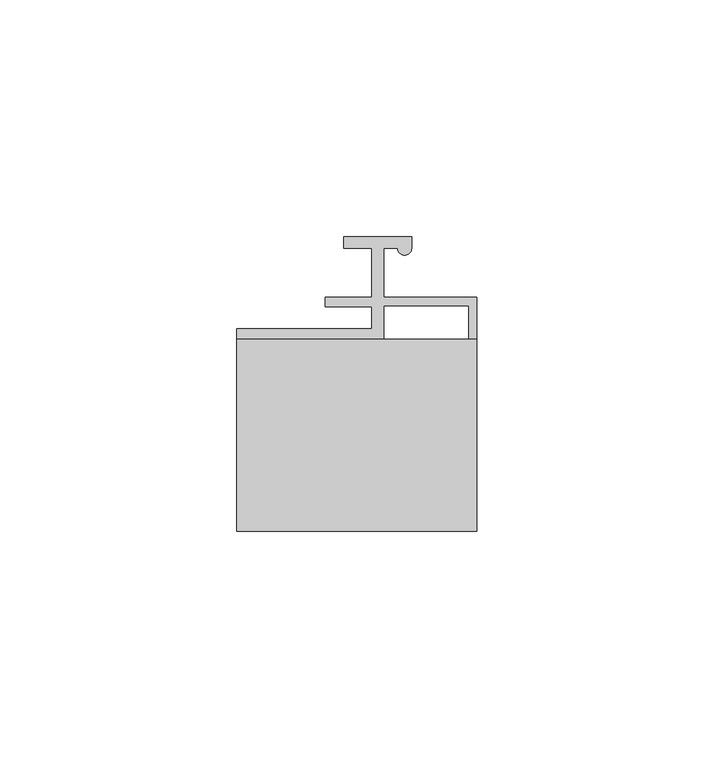
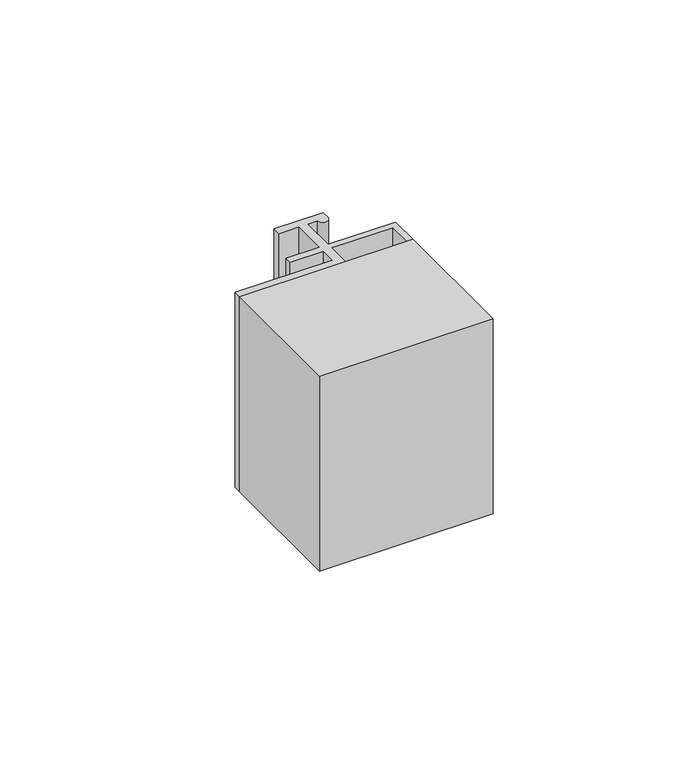
"""IFC4 building model written with IfcOpenShell, lengths in millimetres: proxy geometry, Generic Models 9:Generic Models 5:348123:Generic Models 5:348123 : Generic Models 9:Generic Models 5:348123:1 : Generic Models 9:Generic Models 5:348123:Generic Models 5:348123 : Generic Models 9:Generic Models 5:348123:301771."""

from ifc_helpers import new_model, si_unit, point, frame, frame_2d, origin, place, context, project, spatial, polyline, circle_curve, trimmed, segment, composite_curve, outline, extrude, source, transform, mapped, element, save


def generic_models_7091c7e3(model_context):
    return source(origin(), model_context, "Body", "SweptSolid", [
        extrude(outline(polyline([(30803.1241035, 40787.9731612), (30803.1241035, 40828.5678214), (30853.9241035, 40828.5678214), (30853.9241035, 40787.9731612), (30803.1241035, 40787.9731612)])), frame((0.0, 0.0, 267387.3875), z_axis=(0.0, 0.0, 1.0), x_axis=(1.0, 0.0, 0.0)), (0.0, 0.0, 1.0), 60.325),
        extrude(outline(composite_curve([segment(polyline([(30834.1959481, 40837.4454913), (30853.9241035, 40837.4454913), (30853.9241035, 40828.5678214), (30852.1485695, 40828.5678214), (30852.1485695, 40835.6699573), (30834.1959481, 40835.6699573), (30834.1959481, 40828.5678214), (30803.1241035, 40828.5678214), (30803.1241035, 40830.8365593), (30831.7299287, 40830.8365593), (30831.7299287, 40835.4726758), (30821.8658511, 40835.4726758), (30821.8658511, 40837.4454913), (30831.7299287, 40837.4454913), (30831.7299287, 40847.8027728), (30825.8114821, 40847.8027728), (30825.8114821, 40850.2687923), (30840.1143948, 40850.2687923), (30840.1143948, 40847.8027728)]), True, "CONTINUOUS"), segment(trimmed(circle_curve(frame_2d((30838.6347831, 40847.8027728)), 1.4796117), [point((30840.1143948, 40847.8027728))], [point((30837.1551714, 40847.8027728))], False, "CARTESIAN"), True, "CONTINUOUS"), segment(polyline([(30837.1551714, 40847.8027728), (30834.1959481, 40847.8027728), (30834.1959481, 40837.4454913)]), True, "CONTINUOUS")], self_intersect=False)), frame((0.0, 0.0, 267387.3875), z_axis=(0.0, 0.0, 1.0), x_axis=(1.0, 0.0, 0.0)), (0.0, 0.0, 1.0), 60.325),
    ])


if __name__ == "__main__":
    model = new_model("IFC4")
    model_context = context("Model", 3, world=origin())
    ifc_project = project(units=[si_unit("LENGTHUNIT", "METRE", prefix="MILLI")], contexts=[model_context])
    site = spatial("IfcSite", under=ifc_project)
    building = spatial("IfcBuilding", under=site)
    placement = place(None, origin())
    generic_models_shape = generic_models_7091c7e3(model_context)
    element("IfcBuildingElementProxy", 1, Name="Generic Models 9:Generic Models 5:348123:Generic Models 5:348123 : Generic Models 9:Generic Models 5:348123:1 : Generic Models 9:Generic Models 5:348123:Generic Models 5:348123 : Generic Models 9:Generic Models 5:348123:301771", ObjectType="Generic Models 9:Generic Models 5:348123:Generic Models 5:348123 : Generic Models 9:Generic Models 5:348123:1 : Generic Models 9:Generic Models 5:348123:Generic Models 5:348123 : Generic Models 9:Generic Models 5:348123:301771", at=placement, inside=building, context=model_context, shape_type="MappedRepresentation", body=[
        mapped(generic_models_shape, transform((0.0, 0.0, 0.0), x_axis=(1.0, 0.0, 0.0), y_axis=(0.0, 1.0, 0.0), z_axis=(0.0, 0.0, 1.0))),
    ])
    save(model, "model.ifc")

# Revit data of these elements
# Type "Generic Models 9:Generic Models 5:348123:Generic Models 5:348123 : Generic Models 9:Generic Models 5:348123:1 : Generic Models 9:Generic Models 5:348123:Generic Models 5:348123 : Generic Models 9:Generic Models 5:348123:301771"
#   NameOverride = "Generic Models 9:Generic Models 5:348123:Generic Models 5:348123 : Generic Models 9:Generic Models 5:348123:301771"
#   ObjectTypeOverride = "Generic Models 5:348123 : Generic Models 9:Generic Models 5:348123"
#   Reference = "Generic Models 5"
#   Tag = "301771"
# Element 1 (IfcBuildingElementProxy, "Generic Models 9:Generic Models 5:348123:Generic Models 5:348123 : Generic Models 9:Generic Models 5:348123:1 : Generic Models 9:Generic Models 5:348123:Generic Models 5:348123 : Generic Models 9:Generic Models 5:348123:301771")
#   Materials on its faces: "GA. STEEL CLIP AT EVERY SEAM IN POLYCARBONATE (WITH BLOCKING EXTENSIONS, IF NECS.)"
# Materials
#   "GA. STEEL CLIP AT EVERY SEAM IN POLYCARBONATE (WITH BLOCKING EXTENSIONS, IF NECS.)": class "Unassigned", colour RGB 120 120 120, transparency 0, Cost = 0
